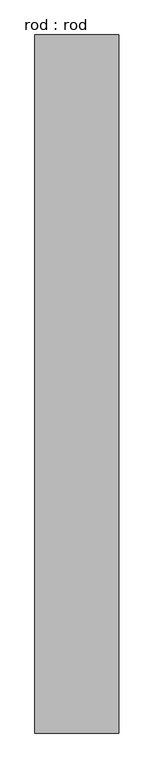
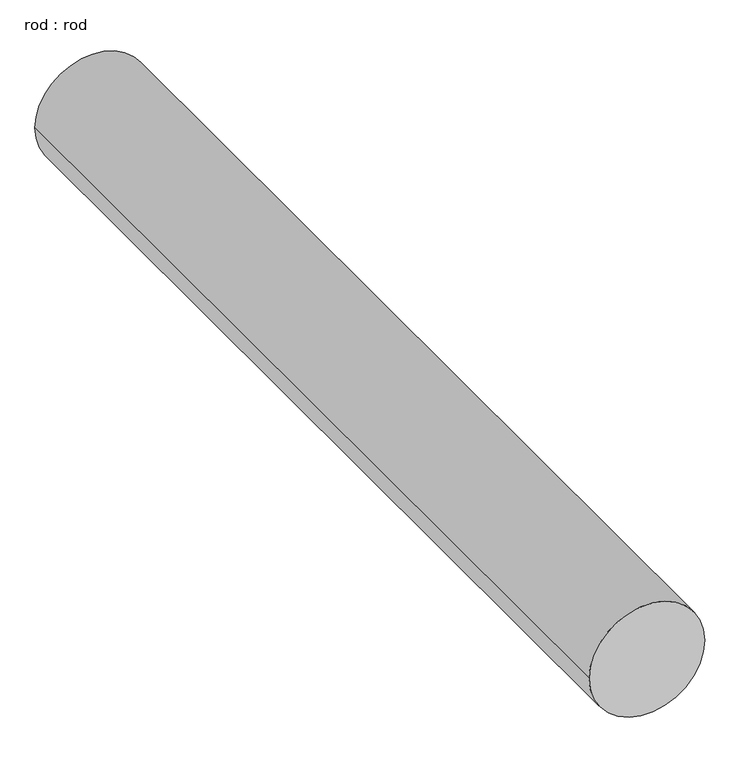
"""IFC4 building model written with IfcOpenShell, lengths in millimetres: proxy geometry, rod : rod."""

from ifc_helpers import new_model, si_unit, point, frame, frame_2d, origin, place, context, project, spatial, circle_curve, trimmed, segment, composite_curve, outline, extrude, source, transform, mapped, element, save


def rod_rod_ce0c95ba(model_context):
    return source(origin(), model_context, "Body", "SweptSolid", [
        extrude(outline(composite_curve([segment(trimmed(circle_curve(frame_2d((0.0108462, 0.0)), 200.0), [point((0.0108462, 200.0))], [point((0.0108462, -200.0))], False, "CARTESIAN"), True, "CONTINUOUS"), segment(trimmed(circle_curve(frame_2d((0.0108462, 0.0)), 200.0), [point((0.0108462, -200.0))], [point((0.0108462, 200.0))], False, "CARTESIAN"), True, "CONTINUOUS")], self_intersect=False)), frame((0.0, 2432.0143296, 0.0), z_axis=(0.0, 1.0, 0.0), x_axis=(0.0, 0.0, 1.0)), (0.0, 0.0, 1.0), 3321.4285714),
    ])


if __name__ == "__main__":
    model = new_model("IFC4")
    model_context = context("Model", 3, world=origin())
    ifc_project = project(units=[si_unit("LENGTHUNIT", "METRE", prefix="MILLI")], contexts=[model_context])
    site = spatial("IfcSite", under=ifc_project)
    building = spatial("IfcBuilding", under=site)
    placement = place(None, origin())
    rod_rod_shape = rod_rod_ce0c95ba(model_context)
    element("IfcBuildingElementProxy", 1, Name="rod : rod", ObjectType="rod : rod", at=placement, inside=building, context=model_context, shape_type="MappedRepresentation", body=[
        mapped(rod_rod_shape, transform((0.0, 0.0, 0.0), x_axis=(1.0, 0.0, 0.0), y_axis=(0.0, 1.0, 0.0), z_axis=(0.0, 0.0, 1.0))),
    ])
    save(model, "model.ifc")

# Revit data of these elements
# Type "rod : rod"
#   Default Elevation = 0
